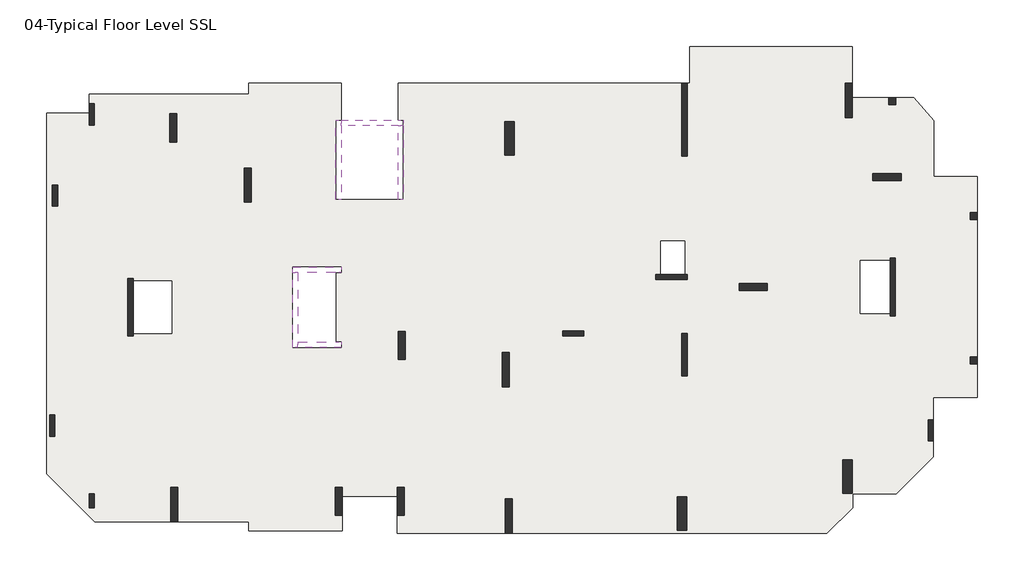
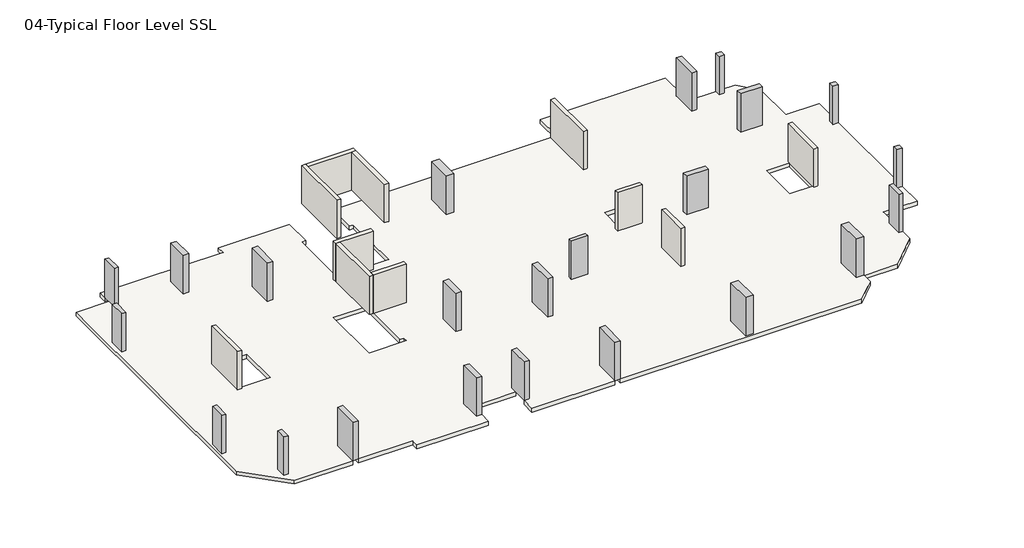
# One storey: 23 columns, 11 walls, 1 slab.
"""IFC4 building model written with IfcOpenShell, lengths in millimetres."""

from ifc_helpers import new_model, si_unit, origin, place, context, project, spatial, faceted_brep, element, save

model = new_model("IFC4")

# Units and contexts
model_context = context("Model", 3, world=origin())
ifc_project = project(units=[si_unit("LENGTHUNIT", "METRE", prefix="MILLI")], contexts=[model_context])

# Site, building, storey
site = spatial("IfcSite", under=ifc_project)
building = spatial("IfcBuilding", under=site)
storey = spatial("IfcBuildingStorey", under=building, Name="04-Typical Floor Level SSL", Elevation=6000.0)

# Columns
placement = place(None, origin())
element("IfcColumn", 1, ObjectType="M_Concrete-Rectangular-Column : C-1 (400 x 400mm)", at=placement, inside=storey, context=model_context, shape_type="Brep", body=[
    faceted_brep([(52549.9999998, 16712.0, 6000.0), (52549.9999998, 16312.0, 6000.0), (52149.9999998, 16312.0, 6000.0), (52149.9999998, 16712.0, 6000.0), (52549.9999998, 16712.0, 9000.0), (52549.9999998, 16312.0, 9000.0), (52549.9999998, 16312.0, 8700.0), (52549.9999998, 16712.0, 8700.0), (52149.9999998, 16312.0, 9000.0), (52149.9999998, 16312.0, 8700.0), (52149.9999998, 16712.0, 9000.0), (52149.9999998, 16712.0, 8700.0)], [[[0, 1, 2, 3]], [[4, 5, 6, 1, 0, 7]], [[5, 8, 9, 2, 1, 6]], [[8, 10, 11, 3, 2, 9]], [[10, 4, 7, 0, 3, 11]], [[4, 10, 8, 5]]]),
])
element("IfcColumn", 2, ObjectType="M_Concrete-Rectangular-Column : C-1 (400 x 400mm)", at=placement, inside=storey, context=model_context, shape_type="Brep", body=[
    faceted_brep([(47898.6337868, 23252.0, 6000.0), (47898.6337868, 22852.0, 6000.0), (47498.6337868, 22852.0, 6000.0), (47498.6337868, 23252.0, 6000.0), (47898.6337868, 23252.0, 9000.0), (47898.6337868, 22852.0, 9000.0), (47898.6337868, 22852.0, 8700.0), (47498.6337868, 22852.0, 9000.0), (47498.6337868, 22852.0, 8700.0), (47498.6337868, 23252.0, 9000.0)], [[[0, 1, 2, 3]], [[4, 5, 6, 1, 0]], [[5, 7, 8, 2, 1, 6]], [[7, 9, 3, 2, 8]], [[9, 4, 0, 3]], [[4, 9, 7, 5]]]),
])
element("IfcColumn", 3, ObjectType="M_Concrete-Rectangular-Column : C-1 (400 x 400mm)", at=placement, inside=storey, context=model_context, shape_type="Brep", body=[
    faceted_brep([(52549.9999998, 8504.0039609, 6000.0), (52549.9999998, 8104.0039609, 6000.0), (52149.9999998, 8104.0039609, 6000.0), (52149.9999998, 8504.0039609, 6000.0), (52549.9999998, 8504.0039609, 9000.0), (52549.9999998, 8104.0039609, 9000.0), (52549.9999998, 8104.0039609, 8700.0), (52549.9999998, 8504.0039609, 8700.0), (52149.9999998, 8104.0039609, 9000.0), (52149.9999998, 8104.0039609, 8700.0), (52149.9999998, 8504.0039609, 9000.0), (52149.9999998, 8504.0039609, 8700.0)], [[[0, 1, 2, 3]], [[4, 5, 6, 1, 0, 7]], [[5, 8, 9, 2, 1, 6]], [[8, 10, 11, 3, 2, 9]], [[10, 4, 7, 0, 3, 11]], [[4, 10, 8, 5]]]),
])
element("IfcColumn", 4, ObjectType="M_Concrete-Rectangular-Column : C-2 (300 x 800mm)", at=placement, inside=storey, context=model_context, shape_type="Brep", body=[
    faceted_brep([(2352.0, 728.0, 6000.0), (2352.0, -72.0, 6000.0), (2052.0, -72.0, 6000.0), (2052.0, 728.0, 6000.0), (2352.0, 728.0, 9000.0), (2352.0, -72.0, 9000.0), (2352.0, -72.0, 8700.0), (2352.0, 728.0, 8700.0), (2052.0, -72.0, 9000.0), (2052.0, -72.0, 8700.0), (2052.0, 728.0, 9000.0), (2052.0, 728.0, 8700.0)], [[[0, 1, 2, 3]], [[4, 5, 6, 1, 0, 7]], [[5, 8, 9, 2, 1, 6]], [[8, 10, 11, 3, 2, 9]], [[10, 4, 7, 0, 3, 11]], [[4, 10, 8, 5]]]),
])
element("IfcColumn", 5, ObjectType="M_Concrete-Rectangular-Column : C-3(300 x 1200mm)", at=placement, inside=storey, context=model_context, shape_type="Brep", body=[
    faceted_brep([(2352.0, 22908.0000656, 6000.0), (2352.0, 21708.0000656, 6000.0), (2052.0, 21708.0000656, 6000.0), (2052.0, 22908.0000656, 6000.0), (2352.0, 22908.0000656, 9000.0), (2352.0, 21708.0000656, 9000.0), (2352.0, 21708.0000656, 8700.0), (2352.0, 22908.0000656, 8700.0), (2052.0, 21708.0000656, 9000.0), (2052.0, 21708.0000656, 8700.0), (2052.0, 22380.0004589, 9000.0), (2052.0, 22908.0000656, 9000.0), (2052.0, 22908.0000656, 8700.0)], [[[0, 1, 2, 3]], [[4, 5, 6, 1, 0, 7]], [[5, 8, 9, 2, 1, 6]], [[8, 10, 11, 12, 3, 2, 9]], [[11, 4, 7, 0, 3, 12]], [[4, 11, 10, 8, 5]]]),
])
element("IfcColumn", 6, ObjectType="M_Concrete-Rectangular-Column : C-3(300 x 1200mm)", at=placement, inside=storey, context=model_context, shape_type="Brep", body=[
    faceted_brep([(257.9999999, 18288.0, 6000.0), (257.9999999, 17088.0, 6000.0), (-42.0000001, 17088.0, 6000.0), (-42.0000001, 18288.0, 6000.0), (257.9999999, 18288.0, 9000.0), (257.9999999, 17088.0, 9000.0), (257.9999999, 17088.0, 8700.0), (257.9999999, 18288.0, 8700.0), (-42.0000001, 17088.0, 9000.0), (-42.0000001, 17088.0, 8700.0), (-42.0000001, 18288.0, 9000.0), (-42.0000001, 18288.0, 8700.0)], [[[0, 1, 2, 3]], [[4, 5, 6, 1, 0, 7]], [[5, 8, 9, 2, 1, 6]], [[8, 10, 11, 3, 2, 9]], [[10, 4, 7, 0, 3, 11]], [[4, 10, 8, 5]]]),
])
element("IfcColumn", 7, ObjectType="M_Concrete-Rectangular-Column : C-3(300 x 1200mm)", at=placement, inside=storey, context=model_context, shape_type="Brep", body=[
    faceted_brep([(108.001803, 5201.9999858, 6000.0), (108.001803, 4001.9999858, 6000.0), (-191.998197, 4001.9999858, 6000.0), (-191.998197, 5201.9999858, 6000.0), (108.001803, 5201.9999858, 9000.0), (108.001803, 4001.9999858, 9000.0), (108.001803, 4001.9999858, 8700.0), (108.001803, 5201.9999858, 8700.0), (-191.998197, 4001.9999858, 9000.0), (-191.998197, 4001.9999858, 8700.0), (-191.998197, 5201.9999858, 9000.0), (-191.998197, 5201.9999858, 8700.0)], [[[0, 1, 2, 3]], [[4, 5, 6, 1, 0, 7]], [[5, 8, 9, 2, 1, 6]], [[8, 10, 11, 3, 2, 9]], [[10, 4, 7, 0, 3, 11]], [[4, 10, 8, 5]]]),
])
element("IfcColumn", 8, ObjectType="M_Concrete-Rectangular-Column : C-3(300 x 1200mm)", at=placement, inside=storey, context=model_context, shape_type="Brep", body=[
    faceted_brep([(50046.0009271, 4931.9999929, 6000.0), (50046.0009271, 3731.9999929, 6000.0), (49746.0009271, 3731.9999929, 6000.0), (49746.0009271, 4931.9999929, 6000.0), (50046.0009271, 4931.9999929, 9000.0), (50046.0009271, 3731.9999929, 9000.0), (50046.0009271, 3731.9999929, 8700.0), (50046.0009271, 4931.9999929, 8700.0), (49746.0009271, 3731.9999929, 9000.0), (49746.0009271, 3731.9999929, 8700.0), (49746.0009271, 4931.9999929, 9000.0), (49746.0009271, 4931.9999929, 8700.0)], [[[0, 1, 2, 3]], [[4, 5, 6, 1, 0, 7]], [[5, 8, 9, 2, 1, 6]], [[8, 10, 11, 3, 2, 9]], [[10, 4, 7, 0, 3, 11]], [[4, 10, 8, 5]]]),
])
element("IfcColumn", 9, ObjectType="M_Concrete-Rectangular-Column : C-3(300 x 1200mm)", at=placement, inside=storey, context=model_context, shape_type="Brep", body=[
    faceted_brep([(28975.9999998, 9996.0000019, 6000.0), (30175.9999998, 9996.0000019, 6000.0), (30175.9999998, 9696.0000019, 6000.0), (28975.9999998, 9696.0000019, 6000.0), (28975.9999998, 9996.0000019, 9000.0), (30175.9999998, 9996.0000019, 9000.0), (30175.9999998, 9996.0000019, 8700.0), (28975.9999998, 9996.0000019, 8700.0), (30175.9999998, 9696.0000019, 9000.0), (30175.9999998, 9696.0000019, 8700.0), (28975.9999998, 9696.0000019, 9000.0), (28975.9999998, 9696.0000019, 8700.0)], [[[0, 1, 2, 3]], [[4, 5, 6, 1, 0, 7]], [[5, 8, 9, 2, 1, 6]], [[8, 10, 11, 3, 2, 9]], [[10, 4, 7, 0, 3, 11]], [[4, 10, 8, 5]]]),
])
element("IfcColumn", 10, ObjectType="M_Concrete-Rectangular-Column : C-4 (400 x 1600mm)", at=placement, inside=storey, context=model_context, shape_type="Brep", body=[
    faceted_brep([(7021.9999999, 22340.0000078, 6000.0), (7021.9999999, 20740.0000078, 6000.0), (6621.9999999, 20740.0000078, 6000.0), (6621.9999999, 22340.0000078, 6000.0), (7021.9999999, 22340.0000078, 9000.0), (7021.9999999, 20740.0000078, 9000.0), (7021.9999999, 20740.0000078, 8700.0), (7021.9999999, 22340.0000078, 8700.0), (6621.9999999, 20740.0000078, 9000.0), (6621.9999999, 20740.0000078, 8700.0), (6621.9999999, 22340.0000078, 9000.0), (6621.9999999, 22340.0000078, 8700.0)], [[[0, 1, 2, 3]], [[4, 5, 6, 1, 0, 7]], [[5, 8, 9, 2, 1, 6]], [[8, 10, 11, 3, 2, 9]], [[10, 4, 7, 0, 3, 11]], [[4, 10, 8, 5]]]),
])
element("IfcColumn", 11, ObjectType="M_Concrete-Rectangular-Column : C-4 (400 x 1600mm)", at=placement, inside=storey, context=model_context, shape_type="Brep", body=[
    faceted_brep([(19969.9997488, 1087.9955348, 6000.0), (19969.9997488, -512.0044652, 6000.0), (19569.9997488, -512.0044652, 6000.0), (19569.9997488, 1087.9955348, 6000.0), (19969.9997488, 1087.9955348, 9000.0), (19969.9997488, -512.0044652, 9000.0), (19969.9997488, -512.0044652, 8700.0), (19969.9997488, 1087.9955348, 8700.0), (19569.9997488, -512.0044652, 9000.0), (19569.9997488, -512.0044652, 8700.0), (19569.9997488, 564.000519, 9000.0), (19569.9997488, 1087.9955348, 9000.0), (19569.9997488, 1087.9955348, 8700.0)], [[[0, 1, 2, 3]], [[4, 5, 6, 1, 0, 7]], [[5, 8, 9, 2, 1, 6]], [[8, 10, 11, 12, 3, 2, 9]], [[11, 4, 7, 0, 3, 12]], [[4, 11, 10, 8, 5]]]),
])
element("IfcColumn", 12, ObjectType="M_Concrete-Rectangular-Column : C-4 (400 x 1600mm)", at=placement, inside=storey, context=model_context, shape_type="Brep", body=[
    faceted_brep([(46605.9993605, 18950.0, 6000.0), (48205.9993605, 18950.0, 6000.0), (48205.9993605, 18550.0, 6000.0), (46605.9993605, 18550.0, 6000.0), (46605.9993605, 18950.0, 9000.0), (48205.9993605, 18950.0, 9000.0), (48205.9993605, 18950.0, 8700.0), (46605.9993605, 18950.0, 8700.0), (48205.9993605, 18550.0, 9000.0), (48205.9993605, 18550.0, 8700.0), (46605.9993605, 18550.0, 9000.0), (46605.9993605, 18550.0, 8700.0)], [[[0, 1, 2, 3]], [[4, 5, 6, 1, 0, 7]], [[5, 8, 9, 2, 1, 6]], [[8, 10, 11, 3, 2, 9]], [[10, 4, 7, 0, 3, 11]], [[4, 10, 8, 5]]]),
])
element("IfcColumn", 13, ObjectType="M_Concrete-Rectangular-Column : C-5 (400 x 1600mm)", at=placement, inside=storey, context=model_context, shape_type="Brep", body=[
    faceted_brep([(20030.000009, 9955.9999979, 6000.0), (20030.000009, 8355.9999979, 6000.0), (19630.000009, 8355.9999979, 6000.0), (19630.000009, 9955.9999979, 6000.0), (20030.000009, 9955.9999979, 9000.0), (20030.000009, 8355.9999979, 9000.0), (20030.000009, 8355.9999979, 8700.0), (20030.000009, 9955.9999979, 8700.0), (19630.000009, 8355.9999979, 9000.0), (19630.000009, 8355.9999979, 8700.0), (19630.000009, 9955.9999979, 9000.0), (19630.000009, 9955.9999979, 8700.0)], [[[0, 1, 2, 3]], [[4, 5, 6, 1, 0, 7]], [[5, 8, 9, 2, 1, 6]], [[8, 10, 11, 3, 2, 9]], [[10, 4, 7, 0, 3, 11]], [[4, 10, 8, 5]]]),
])
element("IfcColumn", 14, ObjectType="M_Concrete-Rectangular-Column : C-5 (400 x 1600mm)", at=placement, inside=storey, context=model_context, shape_type="Brep", body=[
    faceted_brep([(16429.9999981, 1088.0, 6000.0), (16429.9999981, -512.0, 6000.0), (16029.9999981, -512.0, 6000.0), (16029.9999981, 1088.0, 6000.0), (16429.9999981, 1088.0, 9000.0), (16429.9999981, 564.000519, 9000.0), (16429.9999981, -512.0, 9000.0), (16429.9999981, -512.0, 8700.0), (16429.9999981, 1088.0, 8700.0), (16029.9999981, -512.0, 9000.0), (16029.9999981, -512.0, 8700.0), (16029.9999981, 1088.0, 9000.0), (16029.9999981, 1088.0, 8700.0)], [[[0, 1, 2, 3]], [[4, 5, 6, 7, 1, 0, 8]], [[6, 9, 10, 2, 1, 7]], [[9, 11, 12, 3, 2, 10]], [[11, 4, 8, 0, 3, 12]], [[4, 11, 9, 6, 5]]]),
])
element("IfcColumn", 15, ObjectType="M_Concrete-Rectangular-Column : C-5 (400 x 1600mm)", at=placement, inside=storey, context=model_context, shape_type="Brep", body=[
    faceted_brep([(38998.0014887, 12692.0079212, 6000.0), (40598.0014887, 12692.0079212, 6000.0), (40598.0014887, 12292.0079212, 6000.0), (38998.0014887, 12292.0079212, 6000.0), (38998.0014887, 12692.0079212, 9000.0), (40598.0014887, 12692.0079212, 9000.0), (40598.0014887, 12692.0079212, 8700.0), (38998.0014887, 12692.0079212, 8700.0), (40598.0014887, 12292.0079212, 9000.0), (40598.0014887, 12292.0079212, 8700.0), (38998.0014887, 12292.0079212, 9000.0), (38998.0014887, 12292.0079212, 8700.0)], [[[0, 1, 2, 3]], [[4, 5, 6, 1, 0, 7]], [[5, 8, 9, 2, 1, 6]], [[8, 10, 11, 3, 2, 9]], [[10, 4, 7, 0, 3, 11]], [[4, 10, 8, 5]]]),
])
element("IfcColumn", 16, ObjectType="M_Concrete-Rectangular-Column : C-6 (400 x 1950mm)", at=placement, inside=storey, context=model_context, shape_type="Brep", body=[
    faceted_brep([(11270.0000427, 19262.9999996, 6000.0), (11270.0000427, 17312.9999996, 6000.0), (10870.0000427, 17312.9999996, 6000.0), (10870.0000427, 19262.9999996, 6000.0), (11270.0000427, 19262.9999996, 9000.0), (11270.0000427, 17312.9999996, 9000.0), (11270.0000427, 17312.9999996, 8700.0), (11270.0000427, 19262.9999996, 8700.0), (10870.0000427, 17312.9999996, 9000.0), (10870.0000427, 17312.9999996, 8700.0), (10870.0000427, 19262.9999996, 9000.0), (10870.0000427, 19262.9999996, 8700.0)], [[[0, 1, 2, 3]], [[4, 5, 6, 1, 0, 7]], [[5, 8, 9, 2, 1, 6]], [[8, 10, 11, 3, 2, 9]], [[10, 4, 7, 0, 3, 11]], [[4, 10, 8, 5]]]),
])
element("IfcColumn", 17, ObjectType="M_Concrete-Rectangular-Column : C-6 (400 x 1950mm)", at=placement, inside=storey, context=model_context, shape_type="Brep", body=[
    faceted_brep([(7082.0000416, 1083.0000153, 6000.0), (7082.0000416, -866.9999847, 6000.0), (6682.0000416, -866.9999847, 6000.0), (6682.0000416, 1083.0000153, 6000.0), (7082.0000416, 1083.0000153, 9000.0), (7082.0000416, -866.9999847, 9000.0), (7082.0000416, -866.9999847, 8700.0), (7082.0000416, 1083.0000153, 8700.0), (6682.0000416, -866.9999847, 9000.0), (6682.0000416, -866.9999847, 8700.0), (6682.0000416, 1083.0000153, 9000.0), (6682.0000416, 1083.0000153, 8700.0)], [[[0, 1, 2, 3]], [[4, 5, 6, 1, 0, 7]], [[5, 8, 9, 2, 1, 6]], [[8, 10, 11, 3, 2, 9]], [[10, 4, 7, 0, 3, 11]], [[4, 10, 8, 5]]]),
])
element("IfcColumn", 18, ObjectType="M_Concrete-Rectangular-Column : C-6 (400 x 1950mm)", at=placement, inside=storey, context=model_context, shape_type="Brep", body=[
    faceted_brep([(26113.9999998, 422.995535, 6000.0), (26113.9999998, -1527.004465, 6000.0), (25713.9999998, -1527.004465, 6000.0), (25713.9999998, 422.995535, 6000.0), (26113.9999998, 422.995535, 9000.0), (26113.9999998, -1527.004465, 9000.0), (26113.9999998, -1527.004465, 8700.0), (26113.9999998, 422.995535, 8700.0), (25713.9999998, -1527.004465, 9000.0), (25713.9999998, -1527.004465, 8700.0), (25713.9999998, 422.995535, 9000.0), (25713.9999998, 422.995535, 8700.0)], [[[0, 1, 2, 3]], [[4, 5, 6, 1, 0, 7]], [[5, 8, 9, 2, 1, 6]], [[8, 10, 11, 3, 2, 9]], [[10, 4, 7, 0, 3, 11]], [[4, 10, 8, 5]]]),
])
element("IfcColumn", 19, ObjectType="M_Concrete-Rectangular-Column : C-6 (400 x 1950mm)", at=placement, inside=storey, context=model_context, shape_type="Brep", body=[
    faceted_brep([(45446.0007483, 24087.0, 6000.0), (45446.0007483, 22137.0, 6000.0), (45046.0007483, 22137.0, 6000.0), (45046.0007483, 24087.0, 6000.0), (45446.0007483, 24087.0, 9000.0), (45446.0007483, 23252.0000315, 9000.0), (45446.0007483, 22137.0, 9000.0), (45446.0007483, 22137.0, 8700.0), (45446.0007483, 24087.0, 8700.0), (45046.0007483, 22137.0, 9000.0), (45046.0007483, 22137.0, 8700.0), (45046.0007483, 24087.0, 9000.0), (45046.0007483, 24087.0, 8700.0)], [[[0, 1, 2, 3]], [[4, 5, 6, 7, 1, 0, 8]], [[6, 9, 10, 2, 1, 7]], [[9, 11, 12, 3, 2, 10]], [[11, 4, 8, 0, 3, 12]], [[4, 11, 9, 6, 5]]]),
])
element("IfcColumn", 20, ObjectType="M_Concrete-Rectangular-Column : C-6 (400 x 1950mm)", at=placement, inside=storey, context=model_context, shape_type="Brep", body=[
    faceted_brep([(25934.0000455, 8751.0001824, 6000.0), (25934.0000455, 6801.0001824, 6000.0), (25534.0000455, 6801.0001824, 6000.0), (25534.0000455, 8751.0001824, 6000.0), (25934.0000455, 8751.0001824, 9000.0), (25934.0000455, 6801.0001824, 9000.0), (25934.0000455, 6801.0001824, 8700.0), (25934.0000455, 8751.0001824, 8700.0), (25534.0000455, 6801.0001824, 9000.0), (25534.0000455, 6801.0001824, 8700.0), (25534.0000455, 8751.0001824, 9000.0), (25534.0000455, 8751.0001824, 8700.0)], [[[0, 1, 2, 3]], [[4, 5, 6, 1, 0, 7]], [[5, 8, 9, 2, 1, 6]], [[8, 10, 11, 3, 2, 9]], [[10, 4, 7, 0, 3, 11]], [[4, 10, 8, 5]]]),
])
element("IfcColumn", 21, ObjectType="M_Concrete-Rectangular-Column : C-7 (550 x 1900mm)", at=placement, inside=storey, context=model_context, shape_type="Brep", body=[
    faceted_brep([(36035.9999998, 548.0007983, 6000.0), (36035.9999998, -1351.9992017, 6000.0), (35485.9999998, -1351.9992017, 6000.0), (35485.9999998, 548.0007983, 6000.0), (36035.9999998, 548.0007983, 9000.0), (36035.9999998, -1351.9992017, 9000.0), (36035.9999998, -1351.9992017, 8700.0), (36035.9999998, 548.0007983, 8700.0), (35485.9999998, -1351.9992017, 9000.0), (35485.9999998, -1351.9992017, 8700.0), (35485.9999998, 548.0007983, 9000.0), (35485.9999998, 548.0007983, 8700.0)], [[[0, 1, 2, 3]], [[4, 5, 6, 1, 0, 7]], [[5, 8, 9, 2, 1, 6]], [[8, 10, 11, 3, 2, 9]], [[10, 4, 7, 0, 3, 11]], [[4, 10, 8, 5]]]),
])
element("IfcColumn", 22, ObjectType="M_Concrete-Rectangular-Column : C-7 (550 x 1900mm)", at=placement, inside=storey, context=model_context, shape_type="Brep", body=[
    faceted_brep([(45443.9999998, 2648.0, 6000.0), (45443.9999998, 748.0, 6000.0), (44893.9999998, 748.0, 6000.0), (44893.9999998, 2648.0, 6000.0), (45443.9999998, 2648.0, 9000.0), (45443.9999998, 748.0, 9000.0), (45443.9999998, 748.0, 8700.0), (45443.9999998, 2648.0, 8700.0), (44893.9999998, 748.0, 9000.0), (44893.9999998, 748.0, 8700.0), (44893.9999998, 2648.0, 9000.0), (44893.9999998, 2648.0, 8700.0)], [[[0, 1, 2, 3]], [[4, 5, 6, 1, 0, 7]], [[5, 8, 9, 2, 1, 6]], [[8, 10, 11, 3, 2, 9]], [[10, 4, 7, 0, 3, 11]], [[4, 10, 8, 5]]]),
])
element("IfcColumn", 23, ObjectType="M_Concrete-Rectangular-Column : C-7 (550 x 1900mm)", at=placement, inside=storey, context=model_context, shape_type="Brep", body=[
    faceted_brep([(26218.9999998, 21900.0, 6000.0), (26218.9999998, 20000.0, 6000.0), (25668.9999998, 20000.0, 6000.0), (25668.9999998, 21900.0, 6000.0), (26218.9999998, 21900.0, 9000.0), (26218.9999998, 20000.0, 9000.0), (26218.9999998, 20000.0, 8700.0), (26218.9999998, 21900.0, 8700.0), (25668.9999998, 20000.0, 9000.0), (25668.9999998, 20000.0, 8700.0), (25668.9999998, 21900.0, 9000.0), (25668.9999998, 21900.0, 8700.0)], [[[0, 1, 2, 3]], [[4, 5, 6, 1, 0, 7]], [[5, 8, 9, 2, 1, 6]], [[8, 10, 11, 3, 2, 9]], [[10, 4, 7, 0, 3, 11]], [[4, 10, 8, 5]]]),
])

# Slab
element("IfcSlab", 24, ObjectType="Generic 300mm", at=placement, inside=storey, context=model_context, shape_type="Brep", body=[
    faceted_brep([(19619.9997365, 24072.000519, 5700.0), (36192.0021644, 24072.000519, 5700.0), (36192.0021644, 26172.000519, 5700.0), (45446.0007483, 26172.000519, 5700.0), (45446.0007483, 24087.0, 5700.0), (45046.0007483, 24087.0, 5700.0), (45046.0007483, 22137.0, 5700.0), (45446.0007483, 22137.0, 5700.0), (45446.0007483, 23252.0000315, 5700.0), (47498.6337868, 23252.0000315, 5700.0), (47498.6337868, 22852.0, 5700.0), (47898.6337868, 22852.0, 5700.0), (47898.6337868, 23252.0000315, 5700.0), (48936.764334, 23252.0000315, 5700.0), (50076.0016214, 21956.8283806, 5700.0), (50076.0016214, 18780.0084406, 5700.0), (52549.9999998, 18780.0084406, 5700.0), (52549.9999998, 16712.0, 5700.0), (52149.9999998, 16712.0, 5700.0), (52149.9999998, 16312.0, 5700.0), (52549.9999998, 16312.0, 5700.0), (52549.9999998, 8504.0039609, 5700.0), (52149.9999998, 8504.0039609, 5700.0), (52149.9999998, 8104.0039609, 5700.0), (52549.9999998, 8104.0039609, 5700.0), (52549.9999998, 6204.0084406, 5700.0), (50046.0009271, 6204.0084406, 5700.0), (50046.0009271, 4931.9999929, 5700.0), (49746.0009271, 4931.9999929, 5700.0), (49746.0009271, 3731.9999929, 5700.0), (50046.0009271, 3731.9999929, 5700.0), (50046.0009271, 2810.5962809, 5700.0), (47943.4051652, 708.000519, 5700.0), (45456.0017287, 708.000519, 5700.0), (45456.0017287, -61.7051085, 5700.0), (43990.7023722, -1527.004465, 5700.0), (26113.9999998, -1527.004465, 5700.0), (26113.9999998, 422.995535, 5700.0), (25713.9999998, 422.995535, 5700.0), (25713.9999998, -1527.004465, 5700.0), (19569.9997488, -1527.004465, 5700.0), (19569.9997488, -512.0044652, 5700.0), (19969.9997488, -512.0044652, 5700.0), (19969.9997488, 1087.9955348, 5700.0), (19569.9997488, 1087.9955348, 5700.0), (19569.9997488, 564.000519, 5700.0), (16429.9999981, 564.000519, 5700.0), (16429.9999981, 1088.0, 5700.0), (16029.9999981, 1088.0, 5700.0), (16029.9999981, -512.0, 5700.0), (16429.9999981, -512.0, 5700.0), (16429.9999981, -1391.999481, 5700.0), (11136.0000923, -1391.999481, 5700.0), (11136.0000923, -866.9999847, 5700.0), (7082.0000416, -866.9999847, 5700.0), (7082.0000416, 1083.0000153, 5700.0), (6682.0000416, 1083.0000153, 5700.0), (6682.0000416, -866.9999847, 5700.0), (2364.4419097, -866.9999847, 5700.0), (-372.0, 1869.441925, 5700.0), (-372.0, 22380.0004589, 5700.0), (2052.0, 22380.0004589, 5700.0), (2052.0, 21708.0000656, 5700.0), (2352.0, 21708.0000656, 5700.0), (2352.0, 22908.0000656, 5700.0), (2052.0, 22908.0000656, 5700.0), (2052.0, 23472.000519, 5700.0), (11136.0000923, 23472.000519, 5700.0), (11136.0000923, 24072.000519, 5700.0), (16380.0000168, 24072.000519, 5700.0), (16380.0000168, 21972.0, 5700.0), (16079.9999997, 21972.0, 5700.0), (16079.9999997, 21672.0, 5700.0), (16079.9999997, 17468.0, 5700.0), (19919.9999997, 17468.0, 5700.0), (19919.9999997, 21672.0, 5700.0), (19919.9999997, 21972.0, 5700.0), (19619.9997365, 21972.0, 5700.0), (257.9999999, 17088.0, 5700.0), (257.9999999, 18288.0, 5700.0), (-42.0000001, 18288.0, 5700.0), (-42.0000001, 17088.0, 5700.0), (108.001803, 4001.9999858, 5700.0), (108.001803, 5201.9999858, 5700.0), (-191.998197, 5201.9999858, 5700.0), (-191.998197, 4001.9999858, 5700.0), (30175.9999998, 9996.0000019, 5700.0), (28975.9999998, 9996.0000019, 5700.0), (28975.9999998, 9696.0000019, 5700.0), (30175.9999998, 9696.0000019, 5700.0), (7021.9999999, 20740.0000078, 5700.0), (7021.9999999, 22340.0000078, 5700.0), (6621.9999999, 22340.0000078, 5700.0), (6621.9999999, 20740.0000078, 5700.0), (48205.9993605, 18950.0, 5700.0), (46605.9993605, 18950.0, 5700.0), (46605.9993605, 18550.0, 5700.0), (48205.9993605, 18550.0, 5700.0), (20030.000009, 8355.9999979, 5700.0), (20030.000009, 9955.9999979, 5700.0), (19630.000009, 9955.9999979, 5700.0), (19630.000009, 8355.9999979, 5700.0), (11270.0000427, 17312.9999996, 5700.0), (11270.0000427, 19262.9999996, 5700.0), (10870.0000427, 19262.9999996, 5700.0), (10870.0000427, 17312.9999996, 5700.0), (40598.0014887, 12692.0079212, 5700.0), (38998.0014887, 12692.0079212, 5700.0), (38998.0014887, 12292.0079212, 5700.0), (40598.0014887, 12292.0079212, 5700.0), (2352.0, -72.0, 5700.0), (2352.0, 728.0, 5700.0), (2052.0, 728.0, 5700.0), (2052.0, -72.0, 5700.0), (25934.0000455, 6801.0001824, 5700.0), (25934.0000455, 8751.0001824, 5700.0), (25534.0000455, 8751.0001824, 5700.0), (25534.0000455, 6801.0001824, 5700.0), (36035.9999998, -1351.9992017, 5700.0), (36035.9999998, 548.0007983, 5700.0), (35485.9999998, 548.0007983, 5700.0), (35485.9999998, -1351.9992017, 5700.0), (45443.9999998, 748.0, 5700.0), (45443.9999998, 2648.0, 5700.0), (44893.9999998, 2648.0, 5700.0), (44893.9999998, 748.0, 5700.0), (26218.9999998, 20000.0, 5700.0), (26218.9999998, 21900.0, 5700.0), (25668.9999998, 21900.0, 5700.0), (25668.9999998, 20000.0, 5700.0), (16380.0000168, 13620.0000002, 5700.0), (13919.9999907, 13620.0000002, 5700.0), (13619.9999907, 13620.0000002, 5700.0), (13619.9999907, 13320.0000002, 5700.0), (13619.9999907, 9359.999998, 5700.0), (13619.9999907, 9059.999998, 5700.0), (13919.9999907, 9059.999998, 5700.0), (16380.0000168, 9059.999998, 5700.0), (16380.0000168, 9359.999998, 5700.0), (16079.9999907, 9359.999998, 5700.0), (16079.9999907, 13320.0000002, 5700.0), (16380.0000168, 13320.0000002, 5700.0), (4548.0000034, 12840.0000003, 5700.0), (4548.0000034, 9840.0000003, 5700.0), (6743.9999995, 9840.0000003, 5700.0), (6743.9999995, 12840.0000003, 5700.0), (47580.0014798, 13992.0079177, 5700.0), (45900.001729, 13992.0079177, 5700.0), (45900.001729, 10992.0079181, 5700.0), (47580.0014798, 10992.0079181, 5700.0), (35904.002157, 15108.0000083, 5700.0), (34548.0015145, 15108.0000083, 5700.0), (34548.0015145, 13199.9999992, 5700.0), (35904.002157, 13199.9999992, 5700.0), (36192.0021644, 24072.000519, 6000.0), (19619.9997365, 24072.000519, 6000.0), (19619.9997365, 21972.0, 6000.0), (19919.9999997, 21972.0, 6000.0), (19919.9999997, 17468.0, 6000.0), (16079.9999997, 17468.0, 6000.0), (16079.9999997, 21972.0, 6000.0), (16380.0000168, 21972.0, 6000.0), (16380.0000168, 24072.000519, 6000.0), (11136.0000923, 24072.000519, 6000.0), (11136.0000923, 23472.000519, 6000.0), (2052.0, 23472.000519, 6000.0), (2052.0, 22908.0000656, 6000.0), (2352.0, 22908.0000656, 6000.0), (2352.0, 21708.0000656, 6000.0), (2052.0, 21708.0000656, 6000.0), (2052.0, 22380.0004589, 6000.0), (-372.0, 22380.0004589, 6000.0), (-372.0, 1869.441925, 6000.0), (2364.4419097, -866.9999847, 6000.0), (6682.0000416, -866.9999847, 6000.0), (6682.0000416, 1083.0000153, 6000.0), (7082.0000416, 1083.0000153, 6000.0), (7082.0000416, -866.9999847, 6000.0), (11136.0000923, -866.9999847, 6000.0), (11136.0000923, -1391.999481, 6000.0), (16429.9999981, -1391.999481, 6000.0), (16429.9999981, -512.0, 6000.0), (16029.9999981, -512.0, 6000.0), (16029.9999981, 1088.0, 6000.0), (16429.9999981, 1088.0, 6000.0), (16429.9999981, 564.000519, 6000.0), (19569.9997488, 564.000519, 6000.0), (19569.9997488, 1087.9955348, 6000.0), (19969.9997488, 1087.9955348, 6000.0), (19969.9997488, -512.0044652, 6000.0), (19569.9997488, -512.0044652, 6000.0), (19569.9997488, -1527.004465, 6000.0), (25713.9999998, -1527.004465, 6000.0), (25713.9999998, 422.995535, 6000.0), (26113.9999998, 422.995535, 6000.0), (26113.9999998, -1527.004465, 6000.0), (43990.7023722, -1527.004465, 6000.0), (45456.0017287, -61.7051085, 6000.0), (45456.0017287, 708.000519, 6000.0), (47943.4051652, 708.000519, 6000.0), (50046.0009271, 2810.5962809, 6000.0), (50046.0009271, 3731.9999929, 6000.0), (49746.0009271, 3731.9999929, 6000.0), (49746.0009271, 4931.9999929, 6000.0), (50046.0009271, 4931.9999929, 6000.0), (50046.0009271, 6204.0084406, 6000.0), (52549.9999998, 6204.0084406, 6000.0), (52549.9999998, 8104.0039609, 6000.0), (52149.9999998, 8104.0039609, 6000.0), (52149.9999998, 8504.0039609, 6000.0), (52549.9999998, 8504.0039609, 6000.0), (52549.9999998, 16312.0, 6000.0), (52149.9999998, 16312.0, 6000.0), (52149.9999998, 16712.0, 6000.0), (52549.9999998, 16712.0, 6000.0), (52549.9999998, 18780.0084406, 6000.0), (50076.0016214, 18780.0084406, 6000.0), (50076.0016214, 21956.8283806, 6000.0), (48936.764334, 23252.0000315, 6000.0), (47898.6337868, 23252.0000315, 6000.0), (47898.6337868, 22852.0, 6000.0), (47498.6337868, 22852.0, 6000.0), (47498.6337868, 23252.0000315, 6000.0), (45446.0006898, 23252.0000315, 6000.0), (45446.0007483, 22137.0, 6000.0), (45046.0007483, 22137.0, 6000.0), (45046.0007483, 24087.0, 6000.0), (45446.0007483, 24087.0, 6000.0), (45446.0007483, 26172.000519, 6000.0), (36192.0021644, 26172.000519, 6000.0), (257.9999999, 18288.0, 6000.0), (257.9999999, 17088.0, 6000.0), (-42.0000001, 17088.0, 6000.0), (-42.0000001, 18288.0, 6000.0), (108.001803, 5201.9999858, 6000.0), (108.001803, 4001.9999858, 6000.0), (-191.998197, 4001.9999858, 6000.0), (-191.998197, 5201.9999858, 6000.0), (28975.9999998, 9996.0000019, 6000.0), (30175.9999998, 9996.0000019, 6000.0), (30175.9999998, 9696.0000019, 6000.0), (28975.9999998, 9696.0000019, 6000.0), (7021.9999999, 22340.0000078, 6000.0), (7021.9999999, 20740.0000078, 6000.0), (6621.9999999, 20740.0000078, 6000.0), (6621.9999999, 22340.0000078, 6000.0), (46605.9993605, 18950.0, 6000.0), (48205.9993605, 18950.0, 6000.0), (48205.9993605, 18550.0, 6000.0), (46605.9993605, 18550.0, 6000.0), (20030.000009, 9955.9999979, 6000.0), (20030.000009, 8355.9999979, 6000.0), (19630.000009, 8355.9999979, 6000.0), (19630.000009, 9955.9999979, 6000.0), (11270.0000427, 19262.9999996, 6000.0), (11270.0000427, 17312.9999996, 6000.0), (10870.0000427, 17312.9999996, 6000.0), (10870.0000427, 19262.9999996, 6000.0), (38998.0014887, 12692.0079212, 6000.0), (40598.0014887, 12692.0079212, 6000.0), (40598.0014887, 12292.0079212, 6000.0), (38998.0014887, 12292.0079212, 6000.0), (2352.0, 728.0, 6000.0), (2352.0, -72.0, 6000.0), (2052.0, -72.0, 6000.0), (2052.0, 728.0, 6000.0), (25934.0000455, 8751.0001824, 6000.0), (25934.0000455, 6801.0001824, 6000.0), (25534.0000455, 6801.0001824, 6000.0), (25534.0000455, 8751.0001824, 6000.0), (36035.9999998, 548.0007983, 6000.0), (36035.9999998, -1351.9992017, 6000.0), (35485.9999998, -1351.9992017, 6000.0), (35485.9999998, 548.0007983, 6000.0), (45443.9999998, 2648.0, 6000.0), (45443.9999998, 748.0, 6000.0), (44893.9999998, 748.0, 6000.0), (44893.9999998, 2648.0, 6000.0), (26218.9999998, 21900.0, 6000.0), (26218.9999998, 20000.0, 6000.0), (25668.9999998, 20000.0, 6000.0), (25668.9999998, 21900.0, 6000.0), (13619.9999907, 13620.0000002, 6000.0), (16380.0000168, 13620.0000002, 6000.0), (16380.0000168, 13320.0000002, 6000.0), (16079.9999907, 13320.0000002, 6000.0), (16079.9999907, 9359.999998, 6000.0), (16380.0000168, 9359.999998, 6000.0), (16380.0000168, 9059.999998, 6000.0), (13619.9999907, 9059.999998, 6000.0), (4548.0000034, 9840.0000003, 6000.0), (4548.0000034, 12840.0000003, 6000.0), (6743.9999995, 12840.0000003, 6000.0), (6743.9999995, 9840.0000003, 6000.0), (45900.001729, 13992.0079177, 6000.0), (47580.0014798, 13992.0079177, 6000.0), (47580.0014798, 10992.0079181, 6000.0), (45900.001729, 10992.0079181, 6000.0), (34548.0015145, 15108.0000083, 6000.0), (35904.002157, 15108.0000083, 6000.0), (35904.002157, 13199.9999992, 6000.0), (34548.0015145, 13199.9999992, 6000.0)], [[[0, 1, 2, 3, 4, 5, 6, 7, 8, 9, 10, 11, 12, 13, 14, 15, 16, 17, 18, 19, 20, 21, 22, 23, 24, 25, 26, 27, 28, 29, 30, 31, 32, 33, 34, 35, 36, 37, 38, 39, 40, 41, 42, 43, 44, 45, 46, 47, 48, 49, 50, 51, 52, 53, 54, 55, 56, 57, 58, 59, 60, 61, 62, 63, 64, 65, 66, 67, 68, 69, 70, 71, 72, 73, 74, 75, 76, 77], [78, 79, 80, 81], [82, 83, 84, 85], [86, 87, 88, 89], [90, 91, 92, 93], [94, 95, 96, 97], [98, 99, 100, 101], [102, 103, 104, 105], [106, 107, 108, 109], [110, 111, 112, 113], [114, 115, 116, 117], [118, 119, 120, 121], [122, 123, 124, 125], [126, 127, 128, 129], [130, 131, 132, 133, 134, 135, 136, 137, 138, 139, 140, 141], [142, 143, 144, 145], [146, 147, 148, 149], [150, 151, 152, 153]], [[154, 155, 156, 157, 158, 159, 160, 161, 162, 163, 164, 165, 166, 167, 168, 169, 170, 171, 172, 173, 174, 175, 176, 177, 178, 179, 180, 181, 182, 183, 184, 185, 186, 187, 188, 189, 190, 191, 192, 193, 194, 195, 196, 197, 198, 199, 200, 201, 202, 203, 204, 205, 206, 207, 208, 209, 210, 211, 212, 213, 214, 215, 216, 217, 218, 219, 220, 221, 222, 223, 224, 225, 226, 227, 228, 229], [230, 231, 232, 233], [234, 235, 236, 237], [238, 239, 240, 241], [242, 243, 244, 245], [246, 247, 248, 249], [250, 251, 252, 253], [254, 255, 256, 257], [258, 259, 260, 261], [262, 263, 264, 265], [266, 267, 268, 269], [270, 271, 272, 273], [274, 275, 276, 277], [278, 279, 280, 281], [282, 283, 284, 285, 286, 287, 288, 289], [290, 291, 292, 293], [294, 295, 296, 297], [298, 299, 300, 301]], [[69, 162, 161, 70]], [[155, 0, 77, 156]], [[1, 0, 155, 154]], [[2, 1, 154, 229]], [[3, 2, 229, 228]], [[4, 3, 228, 227]], [[218, 13, 12, 219]], [[8, 223, 222, 9]], [[14, 13, 218, 217]], [[15, 14, 217, 216]], [[16, 15, 216, 215]], [[16, 215, 214, 17]], [[206, 25, 24, 207]], [[20, 211, 210, 21]], [[26, 25, 206, 205]], [[26, 205, 204, 27]], [[31, 30, 201, 200]], [[33, 32, 199, 198]], [[34, 33, 198, 197]], [[35, 34, 197, 196]], [[35, 196, 195, 36]], [[191, 40, 39, 192]], [[40, 191, 190, 41]], [[46, 45, 186, 185]], [[180, 51, 50, 181]], [[52, 51, 180, 179]], [[53, 52, 179, 178]], [[53, 178, 177, 54]], [[58, 57, 174, 173]], [[59, 58, 173, 172]], [[60, 59, 172, 171]], [[61, 60, 171, 170]], [[165, 66, 65, 166]], [[67, 66, 165, 164]], [[68, 67, 164, 163]], [[69, 68, 163, 162]], [[63, 168, 167, 64]], [[168, 63, 62, 169]], [[169, 62, 61, 170]], [[64, 167, 166, 65]], [[78, 231, 230, 79]], [[231, 78, 81, 232]], [[232, 81, 80, 233]], [[233, 80, 79, 230]], [[82, 235, 234, 83]], [[235, 82, 85, 236]], [[236, 85, 84, 237]], [[237, 84, 83, 234]], [[29, 202, 201, 30]], [[202, 29, 28, 203]], [[203, 28, 27, 204]], [[86, 239, 238, 87]], [[239, 86, 89, 240]], [[240, 89, 88, 241]], [[241, 88, 87, 238]], [[90, 243, 242, 91]], [[243, 90, 93, 244]], [[244, 93, 92, 245]], [[245, 92, 91, 242]], [[42, 189, 188, 43]], [[189, 42, 41, 190]], [[44, 187, 186, 45]], [[187, 44, 43, 188]], [[94, 247, 246, 95]], [[247, 94, 97, 248]], [[248, 97, 96, 249]], [[249, 96, 95, 246]], [[98, 251, 250, 99]], [[251, 98, 101, 252]], [[252, 101, 100, 253]], [[253, 100, 99, 250]], [[184, 47, 46, 185]], [[49, 182, 181, 50]], [[182, 49, 48, 183]], [[183, 48, 47, 184]], [[102, 255, 254, 103]], [[255, 102, 105, 256]], [[256, 105, 104, 257]], [[257, 104, 103, 254]], [[176, 55, 54, 177]], [[56, 175, 174, 57]], [[175, 56, 55, 176]], [[194, 37, 36, 195]], [[38, 193, 192, 39]], [[193, 38, 37, 194]], [[7, 224, 223, 8]], [[224, 7, 6, 225]], [[5, 226, 225, 6]], [[226, 5, 4, 227]], [[106, 259, 258, 107]], [[259, 106, 109, 260]], [[260, 109, 108, 261]], [[261, 108, 107, 258]], [[110, 263, 262, 111]], [[113, 264, 263, 110]], [[264, 113, 112, 265]], [[265, 112, 111, 262]], [[114, 267, 266, 115]], [[267, 114, 117, 268]], [[268, 117, 116, 269]], [[269, 116, 115, 266]], [[118, 271, 270, 119]], [[271, 118, 121, 272]], [[272, 121, 120, 273]], [[273, 120, 119, 270]], [[122, 275, 274, 123]], [[275, 122, 125, 276]], [[276, 125, 124, 277]], [[277, 124, 123, 274]], [[126, 279, 278, 127]], [[279, 126, 129, 280]], [[280, 129, 128, 281]], [[281, 128, 127, 278]], [[74, 158, 157, 76, 75]], [[284, 141, 140, 285]], [[130, 283, 282, 132, 131]], [[283, 130, 141, 284]], [[138, 287, 286, 139]], [[287, 138, 137, 288]], [[140, 139, 286, 285]], [[132, 282, 289, 135, 134, 133]], [[288, 137, 136, 135, 289]], [[71, 160, 159, 73, 72]], [[160, 71, 70, 161]], [[76, 157, 156, 77]], [[158, 74, 73, 159]], [[142, 291, 290, 143]], [[143, 290, 293, 144]], [[144, 293, 292, 145]], [[291, 142, 145, 292]], [[146, 295, 294, 147]], [[147, 294, 297, 148]], [[148, 297, 296, 149]], [[295, 146, 149, 296]], [[150, 299, 298, 151]], [[151, 298, 301, 152]], [[152, 301, 300, 153]], [[299, 150, 153, 300]], [[32, 31, 200, 199]], [[19, 212, 211, 20]], [[212, 19, 18, 213]], [[213, 18, 17, 214]], [[11, 220, 219, 12]], [[220, 11, 10, 221]], [[221, 10, 9, 222]], [[23, 208, 207, 24]], [[208, 23, 22, 209]], [[209, 22, 21, 210]]]),
])

# Walls
element("IfcWall", 25, ObjectType="Shear Walls 300mm", at=placement, inside=storey, context=model_context, shape_type="Brep", body=[
    faceted_brep([(4548.0000025, 9696.0, 6000.0), (4548.0000025, 12984.0000001, 6000.0), (4548.0000025, 12984.0000001, 8700.0), (4548.0000025, 12984.0000001, 9000.0), (4548.0000025, 12840.0000003, 9000.0), (4548.0000025, 9840.0000003, 9000.0), (4548.0000025, 9696.0, 9000.0), (4548.0000025, 9696.0, 8700.0), (4248.0000025, 9696.0, 6000.0), (4248.0000025, 9696.0, 8700.0), (4248.0000025, 9696.0, 9000.0), (4248.0000025, 12984.0000001, 9000.0), (4248.0000025, 12984.0000001, 8700.0), (4248.0000025, 12984.0000001, 6000.0)], [[[0, 1, 2, 3, 4, 5, 6, 7]], [[8, 9, 10, 11, 12, 13]], [[1, 0, 8, 13]], [[3, 2, 1, 13, 12, 11]], [[6, 5, 4, 3, 11, 10]], [[0, 7, 6, 10, 9, 8]]]),
])
element("IfcWall", 26, ObjectType="Shear Walls 300mm", at=placement, inside=storey, context=model_context, shape_type="Brep", body=[
    faceted_brep([(34248.0015201, 12899.9999992, 6000.0), (36048.0015201, 12899.9999992, 6000.0), (36048.0015201, 12899.9999992, 8700.0), (36048.0015201, 12899.9999992, 9000.0), (34248.0015201, 12899.9999992, 9000.0), (34248.0015201, 12899.9999992, 8700.0), (34248.0015201, 13199.9999992, 6000.0), (34248.0015201, 13199.9999992, 8700.0), (34248.0015201, 13199.9999992, 9000.0), (34548.0015145, 13199.9999992, 9000.0), (35904.002157, 13199.9999992, 9000.0), (36048.0015201, 13199.9999992, 9000.0), (36048.0015201, 13199.9999992, 8700.0), (36048.0015201, 13199.9999992, 6000.0), (35904.002157, 13199.9999992, 6000.0), (34548.0015145, 13199.9999992, 6000.0)], [[[0, 1, 2, 3, 4, 5]], [[6, 7, 8, 9, 10, 11, 12, 13, 14, 15]], [[1, 0, 6, 15, 14, 13]], [[3, 2, 1, 13, 12, 11]], [[4, 3, 11, 10, 9, 8]], [[0, 5, 4, 8, 7, 6]]]),
])
element("IfcWall", 27, ObjectType="Shear Walls 300mm", at=placement, inside=storey, context=model_context, shape_type="Brep", body=[
    faceted_brep([(35748.0054035, 9840.0000002, 6000.0), (35748.0054035, 7428.0000762, 6000.0), (35748.0054035, 7428.0000762, 8700.0), (35748.0054035, 7428.0000762, 9000.0), (35748.0054035, 9840.0000002, 9000.0), (35748.0054035, 9840.0000002, 8700.0), (36048.0054035, 9840.0000002, 6000.0), (36048.0054035, 9840.0000002, 8700.0), (36048.0054035, 9840.0000002, 9000.0), (36048.0054035, 7428.0000762, 9000.0), (36048.0054035, 7428.0000762, 8700.0), (36048.0054035, 7428.0000762, 6000.0)], [[[0, 1, 2, 3, 4, 5]], [[6, 7, 8, 9, 10, 11]], [[1, 0, 6, 11]], [[3, 2, 1, 11, 10, 9]], [[4, 3, 9, 8]], [[0, 5, 4, 8, 7, 6]]]),
])
element("IfcWall", 28, ObjectType="Shear Walls 300mm", at=placement, inside=storey, context=model_context, shape_type="Brep", body=[
    faceted_brep([(47580.0014811, 14136.0000002, 6000.0), (47580.0014811, 10848.0079202, 6000.0), (47580.0014811, 10848.0079202, 8700.0), (47580.0014811, 10848.0079202, 9000.0), (47580.0014811, 10992.0079181, 9000.0), (47580.0014811, 13992.0079177, 9000.0), (47580.0014811, 14136.0000002, 9000.0), (47580.0014811, 14136.0000002, 8700.0), (47880.0014811, 14136.0000002, 6000.0), (47880.0014811, 14136.0000002, 8700.0), (47880.0014811, 14136.0000002, 9000.0), (47880.0014811, 10848.0079202, 9000.0), (47880.0014811, 10848.0079202, 8700.0), (47880.0014811, 10848.0079202, 6000.0)], [[[0, 1, 2, 3, 4, 5, 6, 7]], [[8, 9, 10, 11, 12, 13]], [[1, 0, 8, 13]], [[3, 2, 1, 13, 12, 11]], [[6, 5, 4, 3, 11, 10]], [[0, 7, 6, 10, 9, 8]]]),
])
element("IfcWall", 29, ObjectType="Shear Walls 300mm", at=placement, inside=storey, context=model_context, shape_type="Brep", body=[
    faceted_brep([(36047.9999998, 19932.0, 6000.0), (36047.9999998, 24072.0078999, 6000.0), (36047.9999998, 24072.0078999, 9000.0), (36047.9999998, 19932.0, 9000.0), (36047.9999998, 19932.0, 8700.0), (35747.9999998, 19932.0, 6000.0), (35747.9999998, 19932.0, 8700.0), (35747.9999998, 19932.0, 9000.0), (35747.9999998, 24072.0078999, 9000.0), (35747.9999998, 24072.0078999, 6000.0)], [[[0, 1, 2, 3, 4]], [[5, 6, 7, 8, 9]], [[1, 0, 5, 9]], [[2, 1, 9, 8]], [[3, 2, 8, 7]], [[0, 4, 3, 7, 6, 5]]]),
])
element("IfcWall", 30, ObjectType="Shear Walls 300mm", at=placement, inside=storey, context=model_context, shape_type="Brep", body=[
    faceted_brep([(16379.9999997, 21972.0, 12000.0), (16379.9999997, 21672.0, 12000.0), (16379.9999997, 17468.0, 12000.0), (16379.9999997, 17468.0, 9000.0), (16379.9999997, 21672.0, 9000.0), (16379.9999997, 21972.0, 9000.0), (16079.9999997, 17468.0, 12000.0), (16079.9999997, 21972.0, 12000.0), (16079.9999997, 21972.0, 11700.0), (16079.9999997, 21972.0, 9000.0), (16079.9999997, 17468.0, 9000.0), (16079.9999997, 17468.0, 11700.0)], [[[0, 1, 2, 3, 4, 5]], [[6, 7, 8, 9, 10, 11]], [[2, 1, 0, 7, 6]], [[2, 6, 11, 10, 3]], [[3, 10, 9, 5, 4]], [[0, 5, 9, 8, 7]]]),
])
element("IfcWall", 31, ObjectType="Shear Walls 300mm", at=placement, inside=storey, context=model_context, shape_type="Brep", body=[
    faceted_brep([(16379.9999997, 21972.0, 12000.0), (19619.9997365, 21972.0, 12000.0), (19919.9999997, 21972.0, 12000.0), (19919.9999997, 21972.0, 11700.0), (19919.9999997, 21972.0, 9000.0), (16379.9999997, 21972.0, 9000.0), (19919.9999997, 21672.0, 12000.0), (19619.9999997, 21672.0, 12000.0), (16379.9999997, 21672.0, 12000.0), (16379.9999997, 21672.0, 9000.0), (19619.9999997, 21672.0, 9000.0), (19919.9999997, 21672.0, 9000.0)], [[[0, 1, 2, 3, 4, 5]], [[6, 7, 8, 9, 10, 11]], [[2, 1, 0, 8, 7, 6]], [[8, 0, 5, 9]], [[9, 5, 4, 11, 10]], [[4, 3, 2, 6, 11]]]),
])
element("IfcWall", 32, ObjectType="Shear Walls 300mm", at=placement, inside=storey, context=model_context, shape_type="Brep", body=[
    faceted_brep([(19919.9999997, 21672.0, 12000.0), (19919.9999997, 17468.0, 12000.0), (19919.9999997, 17468.0, 11700.0), (19919.9999997, 17468.0, 9000.0), (19919.9999997, 21672.0, 9000.0), (19619.9999997, 17468.0, 12000.0), (19619.9999997, 21672.0, 12000.0), (19619.9999997, 21672.0, 9000.0), (19619.9999997, 17468.0, 9000.0)], [[[0, 1, 2, 3, 4]], [[5, 6, 7, 8]], [[1, 0, 6, 5]], [[1, 5, 8, 3, 2]], [[6, 0, 4, 7]], [[4, 3, 8, 7]]]),
])
element("IfcWall", 33, ObjectType="Shear Walls 300mm", at=placement, inside=storey, context=model_context, shape_type="Brep", body=[
    faceted_brep([(16380.0000168, 13320.0000002, 12000.0), (16079.9999907, 13320.0000002, 12000.0), (13919.9999907, 13320.0000002, 12000.0), (13619.9999907, 13320.0000002, 12000.0), (13619.9999907, 13320.0000002, 9000.0), (13919.9999907, 13320.0000002, 9000.0), (16380.0000168, 13320.0000002, 9000.0), (16380.0000168, 13320.0000002, 11700.0), (13619.9999907, 13620.0000002, 12000.0), (16380.0000168, 13620.0000002, 12000.0), (16380.0000168, 13620.0000002, 11700.0), (16380.0000168, 13620.0000002, 9000.0), (13619.9999907, 13620.0000002, 9000.0), (13619.9999907, 13620.0000002, 11700.0)], [[[0, 1, 2, 3, 4, 5, 6, 7]], [[8, 9, 10, 11, 12, 13]], [[9, 0, 7, 6, 11, 10]], [[3, 2, 1, 0, 9, 8]], [[11, 6, 5, 4, 12]], [[4, 3, 8, 13, 12]]]),
])
element("IfcWall", 34, ObjectType="Shear Walls 300mm", at=placement, inside=storey, context=model_context, shape_type="Brep", body=[
    faceted_brep([(13919.9999907, 13320.0000002, 12000.0), (13919.9999907, 9359.999998, 12000.0), (13919.9999907, 9059.999998, 12000.0), (13919.9999907, 9059.999998, 9000.0), (13919.9999907, 9359.999998, 9000.0), (13919.9999907, 13320.0000002, 9000.0), (13619.9999907, 9059.999998, 12000.0), (13619.9999907, 13320.0000002, 12000.0), (13619.9999907, 13320.0000002, 9000.0), (13619.9999907, 9059.999998, 9000.0), (13619.9999907, 9059.999998, 11700.0)], [[[0, 1, 2, 3, 4, 5]], [[6, 7, 8, 9, 10]], [[2, 1, 0, 7, 6]], [[7, 0, 5, 8]], [[8, 5, 4, 3, 9]], [[3, 2, 6, 10, 9]]]),
])
element("IfcWall", 35, ObjectType="Shear Walls 300mm", at=placement, inside=storey, context=model_context, shape_type="Brep", body=[
    faceted_brep([(13919.9999907, 9359.999998, 12000.0), (16079.9999907, 9359.999998, 12000.0), (16380.0000168, 9359.999998, 12000.0), (16380.0000168, 9359.999998, 11700.0), (16380.0000168, 9359.999998, 9000.0), (13919.9999907, 9359.999998, 9000.0), (16380.0000168, 9059.999998, 12000.0), (13919.9999907, 9059.999998, 12000.0), (13919.9999907, 9059.999998, 9000.0), (16380.0000168, 9059.999998, 9000.0), (16380.0000168, 9059.999998, 11700.0)], [[[0, 1, 2, 3, 4, 5]], [[6, 7, 8, 9, 10]], [[2, 1, 0, 7, 6]], [[2, 6, 10, 9, 4, 3]], [[7, 0, 5, 8]], [[5, 4, 9, 8]]]),
])

save(model, "model.ifc")

# Revit data of these elements
# Type "M_Concrete-Rectangular-Column : C-1 (400 x 400mm)"
#   Type Mark = "C01"
#   b = 400 mm
#   h = 400 mm
#   Structural Material [instance default] = Concrete, Cast-in-Place gray
# Type "M_Concrete-Rectangular-Column : C-2 (300 x 800mm)"
#   Type Mark = "C02"
#   b = 300 mm
#   h = 800 mm
#   Structural Material [instance default] = Concrete, Cast-in-Place gray
# Type "M_Concrete-Rectangular-Column : C-3(300 x 1200mm)"
#   Type Mark = "C03"
#   b = 300 mm
#   h = 1200 mm
#   Structural Material [instance default] = Concrete, Cast-in-Place gray
# Type "M_Concrete-Rectangular-Column : C-4 (400 x 1600mm)"
#   Type Mark = "C04"
#   b = 400 mm
#   h = 1600 mm
#   Structural Material [instance default] = Concrete, Cast-in-Place gray
# Type "M_Concrete-Rectangular-Column : C-5 (400 x 1600mm)"
#   Type Mark = "C05"
#   b = 400 mm
#   h = 1600 mm
#   Structural Material [instance default] = Concrete, Cast-in-Place gray
# Type "M_Concrete-Rectangular-Column : C-6 (400 x 1950mm)"
#   Type Mark = "C06"
#   b = 400 mm
#   h = 1950 mm
#   Structural Material [instance default] = Concrete, Cast-in-Place gray
# Type "M_Concrete-Rectangular-Column : C-7 (550 x 1900mm)"
#   Type Mark = "C07"
#   b = 550 mm
#   h = 1900 mm
#   Structural Material [instance default] = Concrete, Cast-in-Place gray
# Type "Generic 300mm"
#   Function = 0
#   Layers, outside or top first: 300 mm "Concrete-RC" (function 1)
# Type "Shear Walls 300mm"
#   Layers, outside or top first: 300 mm "Concrete-RC" (function 1)
# Elements 1, 2, 3 (IfcColumn, "M_Concrete-Rectangular-Column : C-1 (400 x 400mm)")
#   Structural Material = Concrete-RC
#   Phase Created = New Construction
#   Materials on its faces: "Concrete-RC"
# Element 4 (IfcColumn, "M_Concrete-Rectangular-Column : C-2 (300 x 800mm)")
#   Structural Material = Concrete-RC
#   Phase Created = New Construction
#   Materials on its faces: "Concrete-RC"
# Elements 5, 6, 7, 8, 9 (IfcColumn, "M_Concrete-Rectangular-Column : C-3(300 x 1200mm)")
#   Structural Material = Concrete-RC
#   Phase Created = New Construction
#   Materials on its faces: "Concrete-RC"
# Elements 10, 11, 12 (IfcColumn, "M_Concrete-Rectangular-Column : C-4 (400 x 1600mm)")
#   Structural Material = Concrete-RC
#   Phase Created = New Construction
#   Materials on its faces: "Concrete-RC"
# Elements 13, 14, 15 (IfcColumn, "M_Concrete-Rectangular-Column : C-5 (400 x 1600mm)")
#   Structural Material = Concrete-RC
#   Phase Created = New Construction
#   Materials on its faces: "Concrete-RC"
# Elements 16, 17, 18, 19, 20 (IfcColumn, "M_Concrete-Rectangular-Column : C-6 (400 x 1950mm)")
#   Structural Material = Concrete-RC
#   Phase Created = New Construction
#   Materials on its faces: "Concrete-RC"
# Elements 21, 22, 23 (IfcColumn, "M_Concrete-Rectangular-Column : C-7 (550 x 1900mm)")
#   Structural Material = Concrete-RC
#   Phase Created = New Construction
#   Materials on its faces: "Concrete-RC"
# Element 24 (IfcSlab, "Generic 300mm")
#   Height Offset From Level = 0 mm
#   built-in parameter 1001954 = 1
#   Phase Created = New Construction
#   Materials on its faces: "Concrete-RC"
# Elements 25, 26, 27, 28, 29 (IfcWall, "Shear Walls 300mm")
#   Top Offset = 0 mm
#   Base Offset = 0 mm
#   wall height = 3000 mm
#   Phase Created = New Construction
#   Base Constraint = 04-Typical Floor Level SSL
#   Top Constraint = 05-Typical Floor Level SSL
#   Materials on its faces: "Concrete-RC"
# Elements 30, 31, 32, 33, 34, 35 (IfcWall, "Shear Walls 300mm")
#   Top Offset = 0 mm
#   Base Offset = 0 mm
#   wall height = 6000 mm
#   Phase Created = New Construction
#   Base Constraint = 04-Typical Floor Level SSL
#   Top Constraint = 06-Typical Floor Level SSL
#   Materials on its faces: "Concrete-RC"
# Materials
#   "Concrete, Cast-in-Place gray": class "Concrete", colour RGB 192 192 192, transparency 0, Description = "Cast-in-place concrete", Cost = 0
#   "Concrete-RC": class "Concrete", colour RGB 128 128 128, transparency 0, Description = "High strength concrete", Cost = 0
